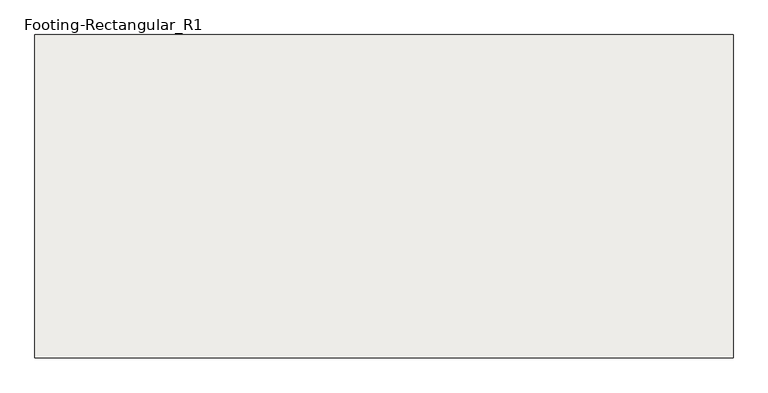
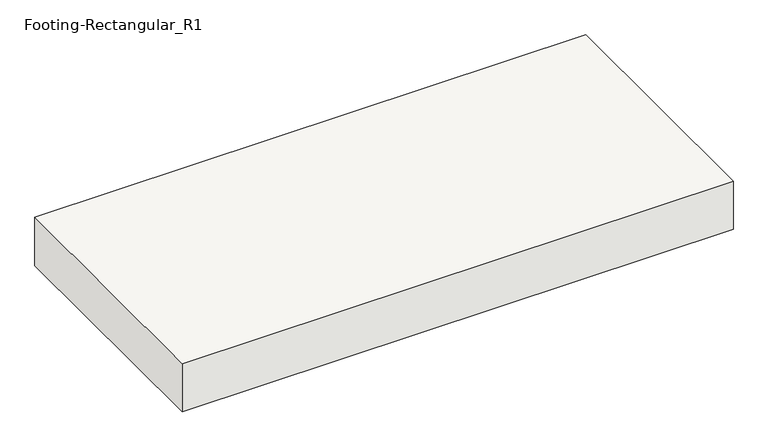
"""IFC4 building model written with IfcOpenShell, lengths in millimetres: slab geometry, Footing-Rectangular_R1 : H_SF_AR_S18_W5400xL2500xT500_Bitumen_F3."""

from ifc_helpers import new_model, si_unit, frame, origin, place, context, project, spatial, polyline, outline, extrude, source, transform, mapped, element, save


def footing_rectangular_r1_ca059662(model_context):
    return source(origin(), model_context, "Body", "SweptSolid", [
        extrude(outline(polyline([(2700.0, 1250.0), (2700.0, -1250.0), (-2700.0, -1250.0), (-2700.0, 1250.0), (2700.0, 1250.0)])), frame((0.0, 0.0, -500.0), z_axis=(0.0, 0.0, 1.0), x_axis=(1.0, 0.0, 0.0)), (0.0, 0.0, 1.0), 500.0),
    ])


if __name__ == "__main__":
    model = new_model("IFC4")
    model_context = context("Model", 3, world=origin())
    ifc_project = project(units=[si_unit("LENGTHUNIT", "METRE", prefix="MILLI")], contexts=[model_context])
    site = spatial("IfcSite", under=ifc_project)
    building = spatial("IfcBuilding", under=site)
    placement = place(None, origin())
    footing_rectangular_r1_shape = footing_rectangular_r1_ca059662(model_context)
    element("IfcSlab", 1, ObjectType="Footing-Rectangular_R1 : H_SF_AR_S18_W5400xL2500xT500_Bitumen_F3", at=placement, inside=building, context=model_context, shape_type="MappedRepresentation", body=[
        mapped(footing_rectangular_r1_shape, transform((0.0, 0.0, 0.0), x_axis=(1.0, 0.0, 0.0), y_axis=(0.0, 1.0, 0.0), z_axis=(0.0, 0.0, 1.0))),
    ])
    save(model, "model.ifc")

# Revit data of these elements
# Type "Footing-Rectangular_R1 : H_SF_AR_S18_W5400xL2500xT500_Bitumen_F3"
#   Type Mark = "F3"
#   Top bar = "D25@300"
#   Description = "UG Shallow Foundation"
#   Bottom bar = "D20@300"
#   Width = 5400 mm
#   Length = 2500 mm
#   Foundation Thickness = 500 mm
#   Structural Material [instance default] = none
#   Assembly Code = ""
